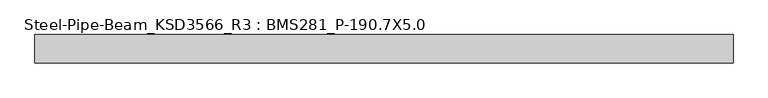
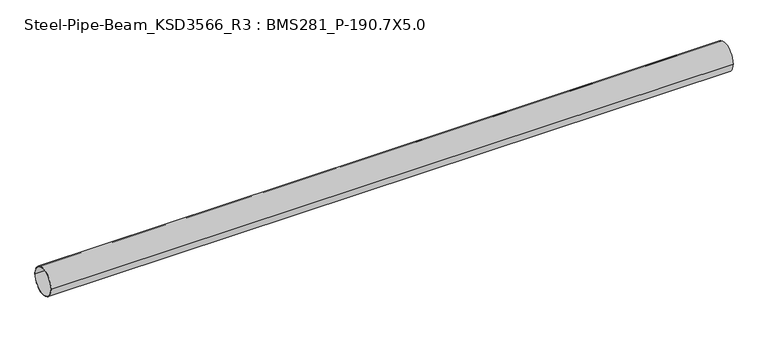
"""IFC4 building model written with IfcOpenShell, lengths in millimetres: member geometry, Steel-Pipe-Beam_KSD3566_R3 : BMS281_P-190.7X5.0."""

from ifc_helpers import new_model, si_unit, point, frame, origin, origin_2d, place, context, project, spatial, circle_curve, trimmed, segment, composite_curve, outline, extrude, source, transform, mapped, element, save


def steel_pipe_beam_ksd3566_r3_bms281_p_190_7x5_0_9db46d87(model_context):
    return source(origin(), model_context, "Body", "SweptSolid", [
        extrude(outline(composite_curve([segment(trimmed(circle_curve(origin_2d(), 95.35), [point((-95.35, 0.0))], [point((95.35, 0.0))], False, "CARTESIAN"), True, "CONTINUOUS"), segment(trimmed(circle_curve(origin_2d(), 95.35), [point((95.35, 0.0))], [point((-95.35, 0.0))], False, "CARTESIAN"), True, "CONTINUOUS")], self_intersect=False), holes=[composite_curve([segment(trimmed(circle_curve(origin_2d(), 90.35), [point((90.35, 0.0))], [point((-90.35, 0.0))], True, "CARTESIAN"), True, "CONTINUOUS"), segment(trimmed(circle_curve(origin_2d(), 90.35), [point((-90.35, 0.0))], [point((90.35, 0.0))], True, "CARTESIAN"), True, "CONTINUOUS")], self_intersect=False)]), frame((-2315.8049318, 0.0, 0.0), z_axis=(1.0, 0.0, 0.0), x_axis=(0.0, 1.0, 0.0)), (0.0, 0.0, 1.0), 4658.0125185),
    ])


if __name__ == "__main__":
    model = new_model("IFC4")
    model_context = context("Model", 3, world=origin())
    ifc_project = project(units=[si_unit("LENGTHUNIT", "METRE", prefix="MILLI")], contexts=[model_context])
    site = spatial("IfcSite", under=ifc_project)
    building = spatial("IfcBuilding", under=site)
    placement = place(None, origin())
    steel_pipe_beam_ksd3566_r3_bms281_p_190_7x5_0_shape = steel_pipe_beam_ksd3566_r3_bms281_p_190_7x5_0_9db46d87(model_context)
    element("IfcMember", 1, ObjectType="Steel-Pipe-Beam_KSD3566_R3 : BMS281_P-190.7X5.0", at=placement, inside=building, context=model_context, shape_type="MappedRepresentation", body=[
        mapped(steel_pipe_beam_ksd3566_r3_bms281_p_190_7x5_0_shape, transform((0.0, 0.0, 0.0), x_axis=(1.0, 0.0, 0.0), y_axis=(0.0, 1.0, 0.0), z_axis=(0.0, 0.0, 1.0))),
    ])
    save(model, "model.ifc")

# Revit data of these elements
# Type "Steel-Pipe-Beam_KSD3566_R3 : BMS281_P-190.7X5.0"
#   Keynote = "P-190.7X5.0"
#   SteelWeight = "Light"
#   t = 0.0050 m
#   Surface Area = 0.599102 m²/m
#   Section Area = 29.1697 cm²
#   Mass per Unit Length = 22.8982 kg/m
#   Length [instance default] = 1.5000 m
#   D = 0.1907 m
#   hec_material4 [instance default] = none
#   hec_material3 [instance default] = none
#   hec_material2 [instance default] = none
#   hec_material1 [instance default] = none
#   Structural Material [instance default] = Steel, 45-345
#   Assembly Code = ""
# Element 1 (IfcMember, "Steel-Pipe-Beam_KSD3566_R3 : BMS281_P-190.7X5.0")
#   Structural Material = none
# Materials
#   "Steel, 45-345": class "Metal", colour RGB 189 187 185, transparency 0, Description = "Steel 345 MPa", Cost = 0
